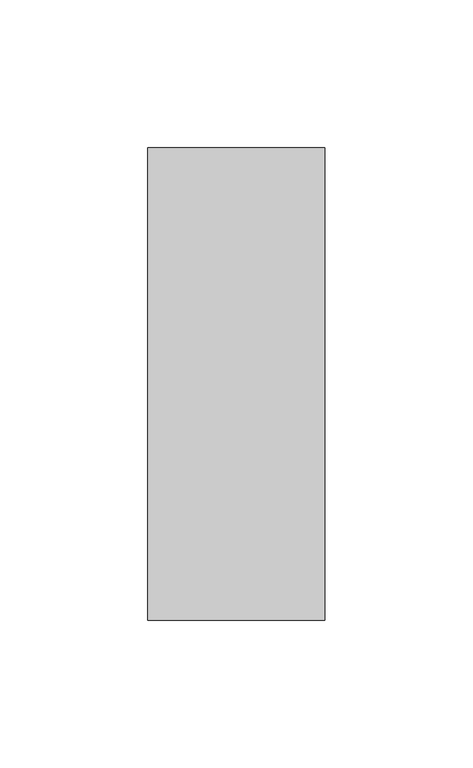
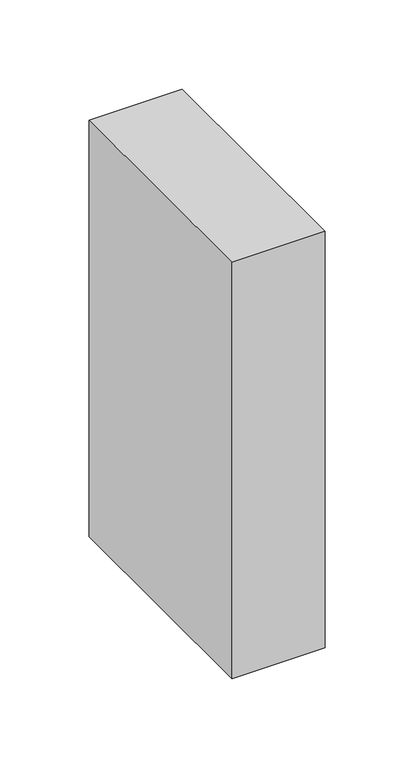
"""IFC4 building model written with IfcOpenShell, lengths in millimetres: column geometry, Madeira de lei-Coluna : Pontalete 6X16cm."""

from ifc_helpers import new_model, si_unit, frame, origin, place, context, project, spatial, polyline, outline, extrude, source, transform, mapped, element, save


def column_1adb463a(model_context):
    return source(origin(), model_context, "Body", "SweptSolid", [
        extrude(outline(polyline([(30.0, 80.0), (30.0, -80.0), (-30.0, -80.0), (-30.0, 80.0), (30.0, 80.0)])), frame((0.0, 0.0, 6710.0), z_axis=(0.0, 0.0, 1.0), x_axis=(1.0, 0.0, 0.0)), (0.0, 0.0, 1.0), 284.6),
    ])


if __name__ == "__main__":
    model = new_model("IFC4")
    model_context = context("Model", 3, world=origin())
    ifc_project = project(units=[si_unit("LENGTHUNIT", "METRE", prefix="MILLI")], contexts=[model_context])
    site = spatial("IfcSite", under=ifc_project)
    building = spatial("IfcBuilding", under=site)
    placement = place(None, origin())
    column_shape = column_1adb463a(model_context)
    element("IfcColumn", 1, ObjectType="Madeira de lei-Coluna : Pontalete 6X16cm", at=placement, inside=building, context=model_context, shape_type="MappedRepresentation", body=[
        mapped(column_shape, transform((0.0, 0.0, 0.0), x_axis=(1.0, 0.0, 0.0), y_axis=(0.0, 1.0, 0.0), z_axis=(0.0, 0.0, 1.0))),
    ])
    save(model, "model.ifc")

# Revit data of these elements
# Type "Madeira de lei-Coluna : Pontalete 6X16cm"
#   A = 0.01952 m²
#   b = 0.06 m
#   d = 0.16 m
#   Structural Material [instance default] = none
#   Assembly Code = ""
# Element 1 (IfcColumn, "Madeira de lei-Coluna : Pontalete 6X16cm")
#   Structural Material = .MADEIRAMENTO
#   Materials on its faces: ".MADEIRAMENTO"
# Materials
#   ".MADEIRAMENTO": class ".CC_MADEIRAS", colour RGB 212 179 113, transparency 0, Cost = 0
